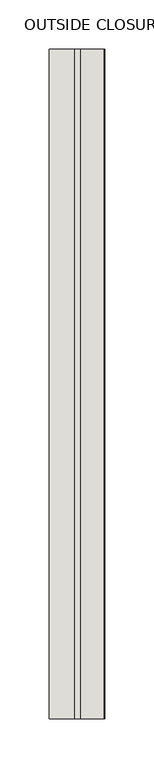
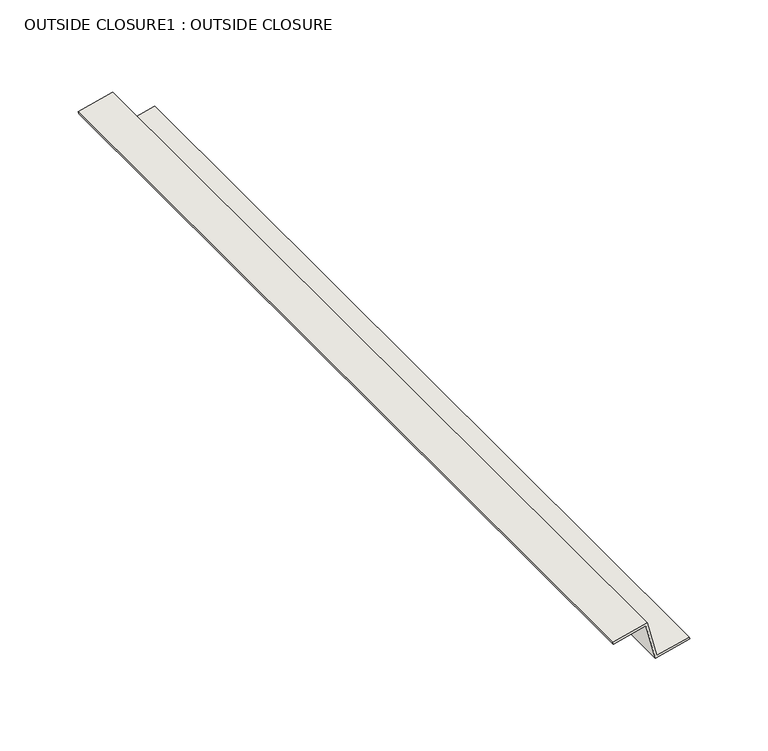
"""IFC4 building model written with IfcOpenShell, lengths in millimetres: wall geometry, OUTSIDE CLOSURE1 : OUTSIDE CLOSURE."""

from ifc_helpers import new_model, si_unit, frame, origin, place, context, project, spatial, polyline, outline, extrude, source, transform, mapped, element, save


def outside_closure1_outside_closure_f88cd990(model_context):
    return source(origin(), model_context, "Body", "SweptSolid", [
        extrude(outline(polyline([(2966.9578938, 19460.1754276), (2965.4177926, 19460.5604529), (2971.3856848, 19484.4320218), (2943.6239737, 19491.3724496), (2949.9768912, 19516.7841197), (2951.5169925, 19516.3990944), (2945.5491002, 19492.5275255), (2973.3108114, 19485.5870977), (2966.9578938, 19460.1754276)])), frame((0.0, -2319.6634634, 0.0), z_axis=(0.0, 1.0, 0.0), x_axis=(0.0, 0.0, 1.0)), (0.0, 0.0, 1.0), 682.625),
    ])


if __name__ == "__main__":
    model = new_model("IFC4")
    model_context = context("Model", 3, world=origin())
    ifc_project = project(units=[si_unit("LENGTHUNIT", "METRE", prefix="MILLI")], contexts=[model_context])
    site = spatial("IfcSite", under=ifc_project)
    building = spatial("IfcBuilding", under=site)
    placement = place(None, origin())
    outside_closure1_outside_closure_shape = outside_closure1_outside_closure_f88cd990(model_context)
    element("IfcWall", 1, ObjectType="OUTSIDE CLOSURE1 : OUTSIDE CLOSURE", at=placement, inside=building, context=model_context, shape_type="MappedRepresentation", body=[
        mapped(outside_closure1_outside_closure_shape, transform((0.0, 0.0, 0.0), x_axis=(1.0, 0.0, 0.0), y_axis=(0.0, 1.0, 0.0), z_axis=(0.0, 0.0, 1.0))),
    ])
    save(model, "model.ifc")

# Revit data of these elements
# Element 1 (IfcWall, "OUTSIDE CLOSURE1 : OUTSIDE CLOSURE")
#   Materials on its faces: "OUTSIDE CLOSURE"
# Materials
#   "OUTSIDE CLOSURE": class "Metal", colour RGB 247 247 247, transparency 0, Cost = 0
